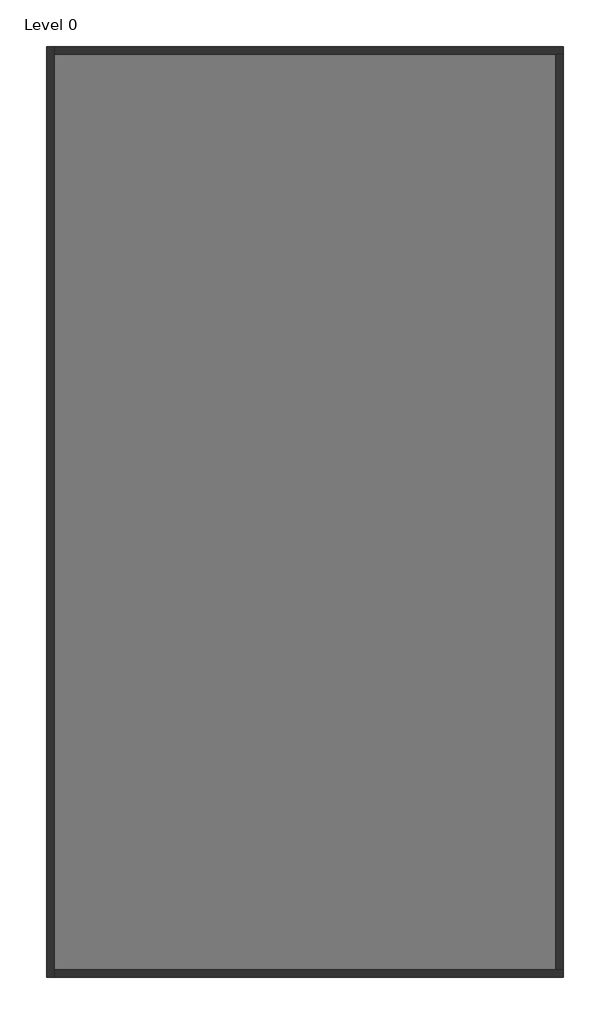
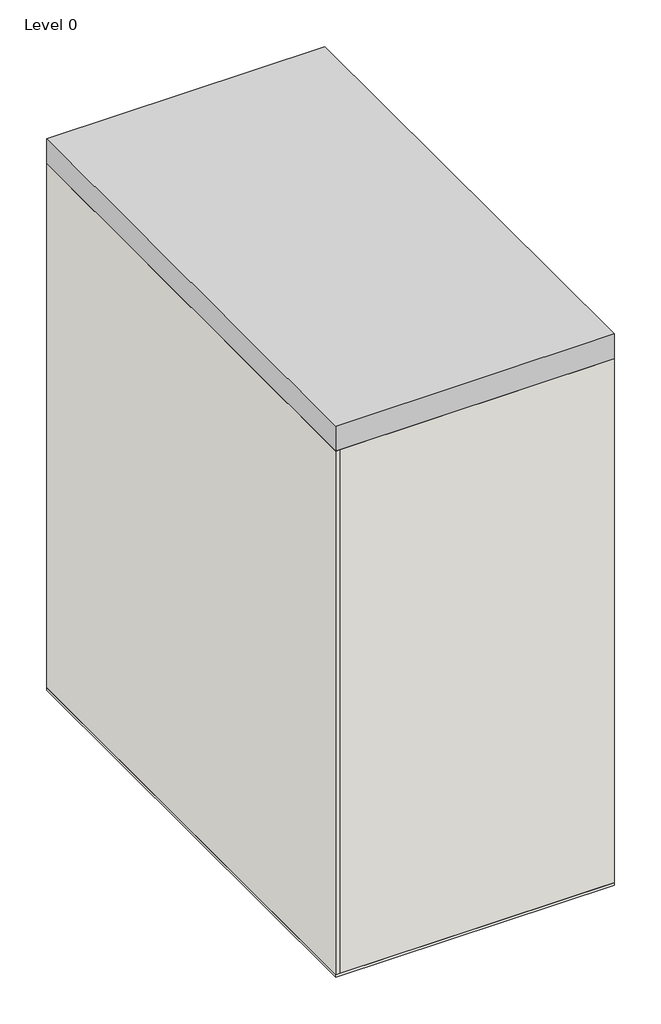
# One storey: 4 walls, 1 proxy, 1 slab.
"""IFC4 building model written with IfcOpenShell, lengths in millimetres."""

from ifc_helpers import new_model, si_unit, frame, origin, origin_with_axes, place, context, project, spatial, polyline, outline, extrude, faceted_brep, element, save

model = new_model("IFC4")

# Units and contexts
model_context = context("Model", 3, world=origin())
ifc_project = project(units=[si_unit("LENGTHUNIT", "METRE", prefix="MILLI")], contexts=[model_context])

# Site, building, storey
site = spatial("IfcSite", under=ifc_project)
building = spatial("IfcBuilding", under=site)
storey = spatial("IfcBuildingStorey", under=building, Name="Level 0", Elevation=100.0)

# Proxy
placement = place(None, origin())
element("IfcBuildingElementProxy", 1, Name="LowUrbanDensityBuilding : LowUrbanDensityBuilding", ObjectType="LowUrbanDensityBuilding : LowUrbanDensityBuilding", at=placement, inside=storey, context=model_context, shape_type="SweptSolid", body=[
    extrude(outline(polyline([(7325.2659446, 3676.2074539), (7325.2659446, -14323.7925461), (-2674.7340554, -14323.7925461), (-2674.7340554, 3676.2074539), (7325.2659446, 3676.2074539)])), origin_with_axes(), (0.0, 0.0, 1.0), 20949.8),
])

# Slab
element("IfcSlab", 2, ObjectType="Floor-Concrete_100Con", at=placement, inside=storey, context=model_context, shape_type="SweptSolid", body=[
    extrude(outline(polyline([(7325.2659446, 3676.2074539), (7325.2659446, -14323.7925461), (-2674.7340554, -14323.7925461), (-2674.7340554, 3676.2074539), (7325.2659446, 3676.2074539)])), origin_with_axes(), (0.0, 0.0, 1.0), 100.0),
])

# Walls
element("IfcWall", 3, ObjectType="Wall-Ext_25Rdr-100Blk-19P", at=placement, inside=storey, context=model_context, shape_type="Brep", body=[
    faceted_brep([(-2674.7340554, 3676.2074539, 100.0), (-2674.7340554, -14323.7925461, 100.0), (-2674.7340554, -14323.7925461, 20000.0), (-2674.7340554, 3676.2074539, 20000.0), (-2530.4340554, 3676.2074539, 100.0), (-2530.4340554, 3676.2074539, 20000.0), (-2530.4340554, 3531.9074539, 20000.0), (-2530.4340554, -14179.4925461, 20000.0), (-2530.4340554, -14323.7925461, 20000.0), (-2530.4340554, -14323.7925461, 100.0), (-2530.4340554, -14179.4925461, 100.0), (-2530.4340554, 3531.9074539, 100.0)], [[[0, 1, 2, 3]], [[4, 5, 6, 7, 8, 9, 10, 11]], [[1, 0, 4, 11, 10, 9]], [[3, 2, 8, 7, 6, 5]], [[2, 1, 9, 8]], [[0, 3, 5, 4]]]),
])
element("IfcWall", 4, ObjectType="Wall-Ext_25Rdr-100Blk-19P", at=placement, inside=storey, context=model_context, shape_type="Brep", body=[
    faceted_brep([(-2530.4340554, -14323.7925461, 100.0), (7325.2659446, -14323.7925461, 100.0), (7325.2659446, -14323.7925461, 20000.0), (-2530.4340554, -14323.7925461, 20000.0), (-2530.4340554, -14179.4925461, 100.0), (-2530.4340554, -14179.4925461, 20000.0), (7180.9659446, -14179.4925461, 20000.0), (7325.2659446, -14179.4925461, 20000.0), (7325.2659446, -14179.4925461, 100.0), (7180.9659446, -14179.4925461, 100.0)], [[[0, 1, 2, 3]], [[4, 5, 6, 7, 8, 9]], [[1, 0, 4, 9, 8]], [[3, 2, 7, 6, 5]], [[0, 3, 5, 4]], [[2, 1, 8, 7]]]),
])
element("IfcWall", 5, ObjectType="Wall-Ext_25Rdr-100Blk-19P", at=placement, inside=storey, context=model_context, shape_type="Brep", body=[
    faceted_brep([(7325.2659446, 3676.2074539, 100.0), (-2530.4340554, 3676.2074539, 100.0), (-2530.4340554, 3676.2074539, 20000.0), (7325.2659446, 3676.2074539, 20000.0), (7325.2659446, 3531.9074539, 100.0), (7325.2659446, 3531.9074539, 20000.0), (7180.9659446, 3531.9074539, 20000.0), (-2530.4340554, 3531.9074539, 20000.0), (-2530.4340554, 3531.9074539, 100.0), (7180.9659446, 3531.9074539, 100.0)], [[[0, 1, 2, 3]], [[4, 5, 6, 7, 8, 9]], [[1, 0, 4, 9, 8]], [[3, 2, 7, 6, 5]], [[2, 1, 8, 7]], [[0, 3, 5, 4]]]),
])
element("IfcWall", 6, ObjectType="Wall-Ext_25Rdr-100Blk-19P", at=placement, inside=storey, context=model_context, shape_type="SweptSolid", body=[
    extrude(outline(polyline([(7325.2659446, 3531.9074539), (7325.2659446, -14179.4925461), (7180.9659446, -14179.4925461), (7180.9659446, 3531.9074539), (7325.2659446, 3531.9074539)])), frame((0.0, 0.0, 100.0), z_axis=(0.0, 0.0, 1.0), x_axis=(1.0, 0.0, 0.0)), (0.0, 0.0, 1.0), 19900.0),
])

save(model, "model.ifc")

# Revit data of these elements
# Project information
#   Project Issue Date = "Issue Date"
#   Project Status = "Project Status"
#   Client Name = "Owner"
#   Project Address = "Enter address here"
#   Project Name = "Project Name"
#   Project Number = "Project Number"
# Type "Floor-Concrete_100Con"
#   Keynote = "E60/130"
#   Function = 0
#   Layers, outside or top first: 100 mm "Concrete" (function 1)
# Type "Wall-Ext_25Rdr-100Blk-19P"
#   Keynote = "F10"
#   Layers, outside or top first: 25.3 mm "Render, Beige, Smooth" (function 5); 100 mm "Concrete Masonry Units _Low Density" (function 1); 19 mm "Plaster" (function 5)
# Element 1 (IfcBuildingElementProxy, "LowUrbanDensityBuilding : LowUrbanDensityBuilding")
#   Phase Created = New Construction
#   Materials on its faces: "Default Form"
# Element 2 (IfcSlab, "Floor-Concrete_100Con")
#   Height Offset From Level = 0 mm
#   Phase Created = New Construction
#   Materials on its faces: "Concrete"
# Element 3 (IfcWall, "Wall-Ext_25Rdr-100Blk-19P")
#   Top Offset = 0 mm
#   Base Offset = 0 mm
#   wall height = 19900 mm
#   Phase Created = New Construction
#   Base Constraint = Level 0
#   Top Constraint = Level 5
#   Materials on its faces: "Render, Beige, Smooth", "Default Wall", "Plaster"
# Elements 4, 5, 6 (IfcWall, "Wall-Ext_25Rdr-100Blk-19P")
#   Top Offset = 0 mm
#   Base Offset = 0 mm
#   wall height = 19900 mm
#   Phase Created = New Construction
#   Base Constraint = Level 0
#   Top Constraint = Level 5
#   Materials on its faces: "Default Wall", "Render, Beige, Smooth", "Plaster"
# Materials
#   "Concrete": class "Concrete", colour RGB 120 120 120, transparency 0, Description = "Portland Cement Concrete", Cost = 0
#   "Render, Beige, Smooth": class "Generic", colour RGB 213 198 180, transparency 0, Description = "physical material", Cost = 0
#   "Concrete Masonry Units _Low Density": class "Masonry", colour RGB 181 181 181, transparency 0, Description = "Concrete masonry units", Cost = 0
#   "Plaster": class "Generic", colour RGB 249 249 249, transparency 0, Description = "Plaster", Cost = 0
#   "Default Form": class "Generic", colour RGB 185 189 196, transparency 0.5, Cost = 0
#   "Default Wall": class "Miscellaneous", colour RGB 128 128 128, transparency 0, Comments = "Rendering appearance not upgraded Rendering appearance not upgraded ", Cost = 0
